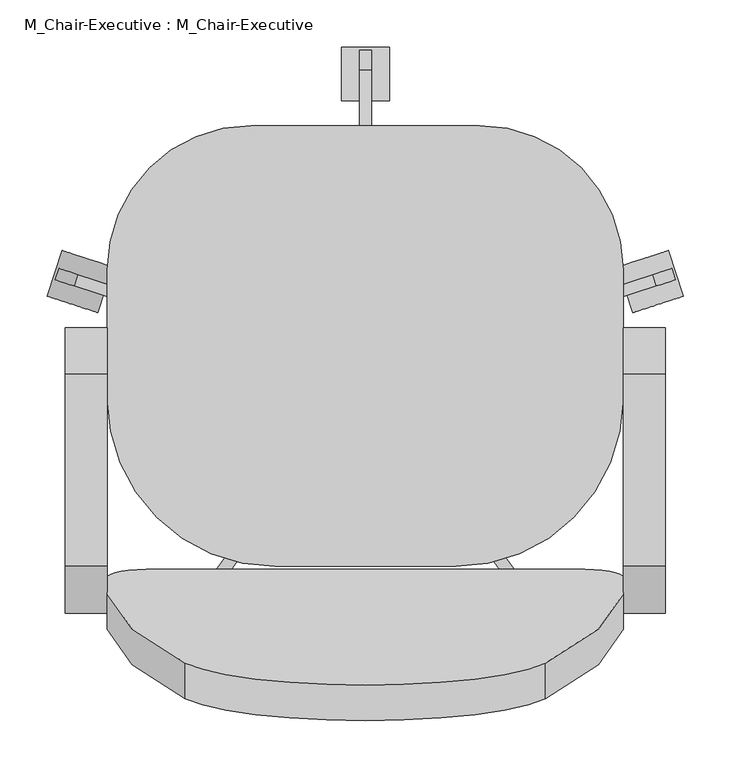
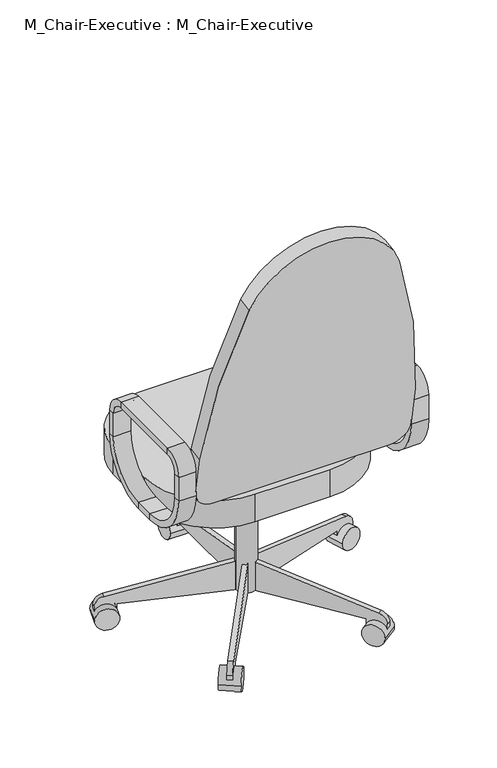
"""IFC4 building model written with IfcOpenShell, lengths in millimetres: furniture geometry, M_Chair-Executive : M_Chair-Executive."""

import ifcopenshell
import ifcopenshell.guid

model = None  # the IFC model being written
_history = None  # IfcOwnerHistory: only IFC2X3 demands one
_inside = {}  # id of a spatial element -> (the spatial element, [elements in it])
_under = {}  # id of a project, library or spatial element -> (it, [spatial elements below it])
_declared = {}  # id of a project -> (the project, [libraries it declares])
_typed = {}  # id of a type object -> (the type object, [elements of that type])
_made_of = {}  # id of a material, layer set ... -> (it, [elements and type objects made of it])


def new_model(schema):
    """Start an empty IFC model of exactly this schema.

    Asked for "IFC4X3", IfcOpenShell would pick the latest addendum, in which some entities
    have other attributes; the version numbers below select the first issue.
    IFC2X3 requires an IfcOwnerHistory on every rooted entity: one is made here for all.
    """
    global model, _history
    if schema == "IFC4X3":
        model = ifcopenshell.file(schema_version=(4, 3, 0, 0))
    else:
        model = ifcopenshell.file(schema=schema)
    _inside.clear()
    _under.clear()
    _declared.clear()
    _typed.clear()
    _made_of.clear()
    _history = None
    if model.schema == "IFC2X3":
        org = make("IfcOrganization", Name="unknown")
        user = make(
            "IfcPersonAndOrganization",
            ThePerson=make("IfcPerson", FamilyName="unknown"),
            TheOrganization=org,
        )
        app = make(
            "IfcApplication",
            ApplicationDeveloper=org,
            Version="unknown",
            ApplicationFullName="unknown",
            ApplicationIdentifier="unknown",
        )
        _history = make(
            "IfcOwnerHistory",
            OwningUser=user,
            OwningApplication=app,
            ChangeAction="ADDED",
            CreationDate=0,
        )
    return model


def make(cls, **values):
    """One entity of the class cls with the attributes given. An attribute that is None is left unset."""
    return model.create_entity(
        cls, **{name: value for name, value in values.items() if value is not None}
    )


def rooted(cls, **values):
    """An entity with a GlobalId (a new one), such as an element, a storey or a relation."""
    return make(cls, GlobalId=ifcopenshell.guid.new(), OwnerHistory=_history, **values)


def si_unit(unit_type, name, prefix=None):
    """IfcSIUnit, for example si_unit("LENGTHUNIT", "METRE", prefix="MILLI")."""
    return make("IfcSIUnit", UnitType=unit_type, Prefix=prefix, Name=name)


def assignment(units):
    """IfcUnitAssignment: the units of a project."""
    return None if units is None else make("IfcUnitAssignment", Units=units)


def point(xyz):
    """IfcCartesianPoint."""
    return None if xyz is None else make("IfcCartesianPoint", Coordinates=xyz)


def direction(xyz):
    """IfcDirection."""
    return None if xyz is None else make("IfcDirection", DirectionRatios=xyz)


def frame(location, z_axis=None, x_axis=None):
    """IfcAxis2Placement3D, a coordinate frame: its origin and axes. An axis left out is left unset."""
    return make(
        "IfcAxis2Placement3D",
        Location=point(location),
        Axis=direction(z_axis),
        RefDirection=direction(x_axis),
    )


def frame_2d(location, x_axis=None):
    """IfcAxis2Placement2D, a coordinate frame in the plane: its origin and x axis."""
    return make(
        "IfcAxis2Placement2D", Location=point(location), RefDirection=direction(x_axis)
    )


def origin():
    """The frame at (0, 0, 0) with its axes left unset."""
    return frame((0.0, 0.0, 0.0))


def place(relative_to, where):
    """IfcLocalPlacement: puts the frame where relative to a parent placement (None: the world)."""
    return make(
        "IfcLocalPlacement", PlacementRelTo=relative_to, RelativePlacement=where
    )


def context(
    kind, dimensions, precision=None, world=None, true_north=None, identifier=None
):
    """IfcGeometricRepresentationContext, for example the 3D "Model" context."""
    return make(
        "IfcGeometricRepresentationContext",
        ContextIdentifier=identifier,
        ContextType=kind,
        CoordinateSpaceDimension=dimensions,
        Precision=precision,
        WorldCoordinateSystem=world,
        TrueNorth=true_north,
    )


def project(units=None, contexts=None):
    """IfcProject with its units and contexts."""
    return rooted(
        "IfcProject",
        Name="project",
        RepresentationContexts=contexts,
        UnitsInContext=assignment(units),
    )


def spatial(cls, under=None, at=None, **own):
    """A site, building, storey or space (cls), placed at a placement, below another one or the project."""
    s = rooted(cls, ObjectPlacement=at, **own)
    if under is not None:
        _under.setdefault(under.id(), (under, []))[1].append(s)
    return s


def polyline(points):
    """IfcPolyline through the points."""
    return make("IfcPolyline", Points=[point(p) for p in points])


def circle_curve(where, radius):
    """IfcCircle in the frame where."""
    return make("IfcCircle", Position=where, Radius=radius)


def trimmed(basis, trim1, trim2, sense, master):
    """IfcTrimmedCurve: the piece of a basis curve between two trims."""
    return make(
        "IfcTrimmedCurve",
        BasisCurve=basis,
        Trim1=trim1,
        Trim2=trim2,
        SenseAgreement=sense,
        MasterRepresentation=master,
    )


def segment(curve, same_sense, transition):
    """IfcCompositeCurveSegment."""
    return make(
        "IfcCompositeCurveSegment",
        Transition=transition,
        SameSense=same_sense,
        ParentCurve=curve,
    )


def composite_curve(segments, self_intersect=None):
    """IfcCompositeCurve: segments joined end to end."""
    return make("IfcCompositeCurve", Segments=segments, SelfIntersect=self_intersect)


def outline(outer, holes=None, kind="AREA"):
    """IfcArbitraryClosedProfileDef: a profile drawn as a closed curve; with holes, ...WithVoids."""
    if holes is None:
        return make("IfcArbitraryClosedProfileDef", ProfileType=kind, OuterCurve=outer)
    return make(
        "IfcArbitraryProfileDefWithVoids",
        ProfileType=kind,
        OuterCurve=outer,
        InnerCurves=holes,
    )


def extrude(swept, where, along, depth):
    """IfcExtrudedAreaSolid: the profile swept, set in the frame where, extruded along a direction by depth."""
    return make(
        "IfcExtrudedAreaSolid",
        SweptArea=swept,
        Position=where,
        ExtrudedDirection=direction(along),
        Depth=depth,
    )


def shape(context_of_items, identifier, shape_type, items):
    """IfcShapeRepresentation: the items that make up one representation, for example the "Body"."""
    return make(
        "IfcShapeRepresentation",
        ContextOfItems=context_of_items,
        RepresentationIdentifier=identifier,
        RepresentationType=shape_type,
        Items=items,
    )


def source(mapping_origin, context_of_items, identifier, shape_type, items):
    """IfcRepresentationMap: a shape defined once, which mapped items show again and again."""
    return make(
        "IfcRepresentationMap",
        MappingOrigin=mapping_origin,
        MappedRepresentation=shape(context_of_items, identifier, shape_type, items),
    )


def transform(
    local_origin,
    x_axis=None,
    y_axis=None,
    z_axis=None,
    scale=None,
    scale2=None,
    scale3=None,
    uniform=True,
):
    """IfcCartesianTransformationOperator3D, or its non-uniform kind. x_axis, y_axis, z_axis: its Axis1, 2, 3."""
    if uniform:
        return make(
            "IfcCartesianTransformationOperator3D",
            Axis1=direction(x_axis),
            Axis2=direction(y_axis),
            LocalOrigin=point(local_origin),
            Scale=scale,
            Axis3=direction(z_axis),
        )
    return make(
        "IfcCartesianTransformationOperator3DnonUniform",
        Axis1=direction(x_axis),
        Axis2=direction(y_axis),
        LocalOrigin=point(local_origin),
        Scale=scale,
        Axis3=direction(z_axis),
        Scale2=scale2,
        Scale3=scale3,
    )


def mapped(mapping_source, mapping_target):
    """IfcMappedItem: shows the shape of a source again, moved by a transform."""
    return make(
        "IfcMappedItem", MappingSource=mapping_source, MappingTarget=mapping_target
    )


def made_of(thing, what):
    """Note that an element or type object is made of a material, layer set ...; save() writes the relation."""
    if what is not None:
        _made_of.setdefault(what.id(), (what, []))[1].append(thing)
    return thing


def element(
    cls,
    number,
    at=None,
    inside=None,
    cuts=None,
    type_object=None,
    material=None,
    context=None,
    identifier="Body",
    shape_type=None,
    held_by="IfcProductDefinitionShape",
    body=None,
    shapes=None,
    **own,
):
    """One element of the class cls, such as IfcWall. Its Tag is "e" and its number.

    at: its placement. inside: the storey or other place that contains it. cuts: it is an
    opening in that element (IfcRelVoidsElement). A single representation is given by context,
    identifier, shape_type and body (its items); several are given by shapes. held_by: the class
    of the entity that holds the representations. save() writes the other relations.
    """
    e = rooted(cls, Tag="e%d" % number, ObjectPlacement=at, **own)
    if body is not None:
        shapes = [shape(context, identifier, shape_type, body)]
    if shapes is not None:
        e.Representation = make(held_by, Representations=shapes)
    if inside is not None:
        _inside.setdefault(inside.id(), (inside, []))[1].append(e)
    if cuts is not None:
        rooted(
            "IfcRelVoidsElement", RelatingBuildingElement=cuts, RelatedOpeningElement=e
        )
    if type_object is not None:
        _typed.setdefault(type_object.id(), (type_object, []))[1].append(e)
    return made_of(e, material)


def aggregate(whole, parts):
    """IfcRelAggregates: a whole, such as a stair, and the parts it consists of."""
    return rooted("IfcRelAggregates", RelatingObject=whole, RelatedObjects=parts)


def save(model, path):
    """Write the relations noted so far, then the file.

    IfcRelAggregates (storeys below a building ...), IfcRelContainedInSpatialStructure (elements
    in a storey), IfcRelDefinesByType, IfcRelAssociatesMaterial and IfcRelDeclares: one each for
    every whole, place, type object, material and project.
    """
    for whole, parts in _under.values():
        aggregate(whole, parts)
    for where, things in _inside.values():
        rooted(
            "IfcRelContainedInSpatialStructure",
            RelatedElements=things,
            RelatingStructure=where,
        )
    for kind, things in _typed.values():
        rooted("IfcRelDefinesByType", RelatedObjects=things, RelatingType=kind)
    for what, things in _made_of.values():
        rooted("IfcRelAssociatesMaterial", RelatedObjects=things, RelatingMaterial=what)
    for by, libraries in _declared.values():
        rooted("IfcRelDeclares", RelatingContext=by, RelatedDefinitions=libraries)
    model.write(path)


def plane_surface(at):
    """IfcPlane: the flat surface through the origin of the frame at, square to its z axis."""
    return make("IfcPlane", Position=at)


def cylinder_surface(at, radius):
    """IfcCylindricalSurface: all points at the distance radius from the z axis of the frame at."""
    return make("IfcCylindricalSurface", Position=at, Radius=radius)


def revolved_surface(curve, axis_point, axis_direction):
    """IfcSurfaceOfRevolution: the curve turned about the line through axis_point along axis_direction."""
    return make(
        "IfcSurfaceOfRevolution",
        SweptCurve=make("IfcArbitraryOpenProfileDef", ProfileType="CURVE", Curve=curve),
        AxisPosition=make("IfcAxis1Placement", Location=point(axis_point), Axis=direction(axis_direction)),
    )


def advanced_brep(points, edges, surfaces, faces):
    """IfcAdvancedBrep: a solid bounded by faces that lie on surfaces and meet in shared edges.

    An edge is (start, end): straight between two places in points (the first is 0);
    or (start, end, curve); or (start, end, curve, False) where it runs against its curve.
    A face is (place in surfaces, loops), or (place, loops, False) where it looks against
    its surface's normal. A loop lists edges by number (the first is 1), with a minus sign
    where the edge is run from its end to its start. The first loop is the outer one.
    """
    corners = [point(p) for p in points]
    vertices = [make("IfcVertexPoint", VertexGeometry=c) for c in corners]
    made = []
    for start, end, *more in edges:
        made.append(
            make(
                "IfcEdgeCurve",
                EdgeStart=vertices[start],
                EdgeEnd=vertices[end],
                EdgeGeometry=more[0] if more else make("IfcPolyline", Points=[corners[start], corners[end]]),
                SameSense=more[1] if len(more) > 1 else True,
            )
        )
    hull = []
    for where, loops, *sense in faces:
        bounds = []
        for j, loop in enumerate(loops):
            ring = [make("IfcOrientedEdge", EdgeElement=made[abs(k) - 1], Orientation=k > 0) for k in loop]
            bounds.append(
                make(
                    "IfcFaceOuterBound" if j == 0 else "IfcFaceBound",
                    Bound=make("IfcEdgeLoop", EdgeList=ring),
                    Orientation=True,
                )
            )
        hull.append(make("IfcAdvancedFace", Bounds=bounds, FaceSurface=surfaces[where], SameSense=sense[0] if sense else True))
    return make("IfcAdvancedBrep", Outer=make("IfcClosedShell", CfsFaces=hull))


def m_chair_executive_m_chair_executive_8d69e98c(model_context):
    return source(origin(), model_context, "Body", "SolidModel", [
        advanced_brep(
        [(-176.5091803, -217.7873012, 546.1), (-176.5091803, -108.0540984, 436.3667972), (-176.5091803, -108.0540984, 420.4917972), (-176.5091803, -233.6623012, 546.1), (-132.0591803, -217.7873012, 546.1), (-132.0591803, -108.0540984, 436.3667972), (-132.0591803, -233.6623012, 546.1), (-132.0591803, -108.0540984, 420.4917972), (-176.5091803, -233.6623012, 609.6), (-176.5091803, -217.7873012, 609.6), (-132.0591803, -217.7873012, 609.6), (-132.0591803, -233.6623012, 609.6), (-176.5091803, -184.2540984, 643.1332028), (-176.5091803, -184.2540984, 659.0082028), (-132.0591803, -184.2540984, 643.1332028), (-132.0591803, -184.2540984, 659.0082028), (-176.5091803, 18.9459016, 659.0082028), (-176.5091803, 18.9459016, 643.1332028), (-132.0591803, 18.9459016, 643.1332028), (-132.0591803, 18.9459016, 659.0082028), (-176.5091803, 52.4791044, 609.6), (-176.5091803, 68.3541044, 609.6), (-132.0591803, 52.4791044, 609.6), (-132.0591803, 68.3541044, 609.6), (-176.5091803, 68.3541044, 546.1), (-176.5091803, 52.4791044, 546.1), (-132.0591803, 52.4791044, 546.1), (-132.0591803, 68.3541044, 546.1), (-176.5091803, -57.2540984, 436.3667972), (-176.5091803, -57.2540984, 420.4917972), (-132.0591803, -57.2540984, 436.3667972), (-132.0591803, -57.2540984, 420.4917972)],
        [
            (0, 1, circle_curve(frame((-176.5091803, -108.0540984, 546.1), z_axis=(1.0, 0.0, 0.0), x_axis=(0.0, 0.0, -1.0)), 109.7332028)),
            (1, 2),
            (2, 3, circle_curve(frame((-176.5091803, -108.0540984, 546.1), z_axis=(-1.0, 0.0, 0.0), x_axis=(0.0, 0.0, -1.0)), 125.6082028)),
            (3, 0),
            (4, 5, circle_curve(frame((-132.0591803, -108.0540984, 546.1), z_axis=(1.0, 0.0, 0.0), x_axis=(0.0, 0.0, -1.0)), 109.7332028)),
            (5, 1),
            (0, 4),
            (6, 7, circle_curve(frame((-132.0591803, -108.0540984, 546.1), z_axis=(1.0, 0.0, 0.0), x_axis=(0.0, 0.0, -1.0)), 125.6082028)),
            (7, 5),
            (4, 6),
            (2, 7),
            (6, 3),
            (3, 8),
            (8, 9),
            (9, 0),
            (9, 10),
            (10, 4),
            (10, 11),
            (11, 6),
            (11, 8),
            (12, 9, circle_curve(frame((-176.5091803, -184.2540984, 609.6), z_axis=(1.0, 0.0, 0.0), x_axis=(0.0, -1.0, 0.0)), 33.5332028)),
            (8, 13, circle_curve(frame((-176.5091803, -184.2540984, 609.6), z_axis=(-1.0, 0.0, 0.0), x_axis=(0.0, -1.0, 0.0)), 49.4082028)),
            (13, 12),
            (14, 10, circle_curve(frame((-132.0591803, -184.2540984, 609.6), z_axis=(1.0, 0.0, 0.0), x_axis=(0.0, -1.0, 0.0)), 33.5332028)),
            (12, 14),
            (15, 11, circle_curve(frame((-132.0591803, -184.2540984, 609.6), z_axis=(1.0, 0.0, 0.0), x_axis=(0.0, -1.0, 0.0)), 49.4082028)),
            (14, 15),
            (15, 13),
            (13, 16),
            (16, 17),
            (17, 12),
            (17, 18),
            (18, 14),
            (18, 19),
            (19, 15),
            (19, 16),
            (20, 17, circle_curve(frame((-176.5091803, 18.9459016, 609.6), z_axis=(1.0, 0.0, 0.0), x_axis=(0.0, 0.0, 1.0)), 33.5332028)),
            (16, 21, circle_curve(frame((-176.5091803, 18.9459016, 609.6), z_axis=(-1.0, 0.0, 0.0), x_axis=(0.0, 0.0, 1.0)), 49.4082028)),
            (21, 20),
            (22, 18, circle_curve(frame((-132.0591803, 18.9459016, 609.6), z_axis=(1.0, 0.0, 0.0), x_axis=(0.0, 0.0, 1.0)), 33.5332028)),
            (20, 22),
            (23, 19, circle_curve(frame((-132.0591803, 18.9459016, 609.6), z_axis=(1.0, 0.0, 0.0), x_axis=(0.0, 0.0, 1.0)), 49.4082028)),
            (22, 23),
            (23, 21),
            (21, 24),
            (24, 25),
            (25, 20),
            (25, 26),
            (26, 22),
            (26, 27),
            (27, 23),
            (27, 24),
            (28, 25, circle_curve(frame((-176.5091803, -57.2540984, 546.1), z_axis=(1.0, 0.0, 0.0), x_axis=(0.0, 1.0, 0.0)), 109.7332028)),
            (24, 29, circle_curve(frame((-176.5091803, -57.2540984, 546.1), z_axis=(-1.0, 0.0, 0.0), x_axis=(0.0, 1.0, 0.0)), 125.6082028)),
            (29, 28),
            (30, 26, circle_curve(frame((-132.0591803, -57.2540984, 546.1), z_axis=(1.0, 0.0, 0.0), x_axis=(0.0, 1.0, 0.0)), 109.7332028)),
            (28, 30),
            (31, 27, circle_curve(frame((-132.0591803, -57.2540984, 546.1), z_axis=(1.0, 0.0, 0.0), x_axis=(0.0, 1.0, 0.0)), 125.6082028)),
            (30, 31),
            (31, 29),
            (29, 2),
            (1, 28),
            (5, 30),
            (7, 31),
        ],
        [
            plane_surface(frame((-176.5091803, -108.0540984, 546.1), z_axis=(-1.0, 0.0, 0.0), x_axis=(0.0, 0.0, -1.0))),
            revolved_surface(polyline([(-176.5091803, -108.0540984, 436.3667972), (-132.0591803, -108.0540984, 436.3667972)]), (-132.0591803, -108.0540984, 546.1), (-1.0, 0.0, 0.0)),
            plane_surface(frame((-132.0591803, -108.0540984, 546.1), z_axis=(1.0, 0.0, 0.0), x_axis=(0.0, 0.0, -1.0))),
            cylinder_surface(frame((-132.0591803, -108.0540984, 546.1), z_axis=(-1.0, 0.0, 0.0), x_axis=(0.0, 0.0, -1.0)), 125.6082028),
            plane_surface(frame((-176.5091803, -233.6623012, 546.1), z_axis=(-1.0, 0.0, 0.0), x_axis=(0.0, 0.0, 1.0))),
            plane_surface(frame((-176.5091803, -217.7873012, 546.1), z_axis=(0.0, 1.0, 0.0), x_axis=(0.0, 0.0, 1.0))),
            plane_surface(frame((-132.0591803, -217.7873012, 546.1), z_axis=(1.0, 0.0, 0.0), x_axis=(0.0, 0.0, 1.0))),
            plane_surface(frame((-132.0591803, -233.6623012, 546.1), z_axis=(0.0, -1.0, 0.0), x_axis=(0.0, 0.0, 1.0))),
            plane_surface(frame((-176.5091803, -184.2540984, 609.6), z_axis=(-1.0, 0.0, 0.0), x_axis=(0.0, -1.0, 0.0))),
            revolved_surface(polyline([(-176.5091803, -217.7873012, 609.6), (-132.0591803, -217.7873012, 609.6)]), (-132.0591803, -184.2540984, 609.6), (-1.0, 0.0, 0.0)),
            plane_surface(frame((-132.0591803, -184.2540984, 609.6), z_axis=(1.0, 0.0, 0.0), x_axis=(0.0, -1.0, 0.0))),
            cylinder_surface(frame((-132.0591803, -184.2540984, 609.6), z_axis=(-1.0, 0.0, 0.0), x_axis=(0.0, -1.0, 0.0)), 49.4082028),
            plane_surface(frame((-176.5091803, -184.2540984, 659.0082028), z_axis=(-1.0, 0.0, 0.0), x_axis=(0.0, 1.0, 0.0))),
            plane_surface(frame((-176.5091803, -184.2540984, 643.1332028), z_axis=(0.0, 0.0, -1.0), x_axis=(0.0, 1.0, 0.0))),
            plane_surface(frame((-132.0591803, -184.2540984, 643.1332028), z_axis=(1.0, 0.0, 0.0), x_axis=(0.0, 1.0, 0.0))),
            plane_surface(frame((-132.0591803, -184.2540984, 659.0082028), z_axis=(0.0, 0.0, 1.0), x_axis=(0.0, 1.0, 0.0))),
            plane_surface(frame((-176.5091803, 18.9459016, 609.6), z_axis=(-1.0, 0.0, 0.0), x_axis=(0.0, 0.0, 1.0))),
            revolved_surface(polyline([(-176.5091803, 18.9459016, 643.1332028), (-132.0591803, 18.9459016, 643.1332028)]), (-132.0591803, 18.9459016, 609.6), (-1.0, 0.0, 0.0)),
            plane_surface(frame((-132.0591803, 18.9459016, 609.6), z_axis=(1.0, 0.0, 0.0), x_axis=(0.0, 0.0, 1.0))),
            cylinder_surface(frame((-132.0591803, 18.9459016, 609.6), z_axis=(-1.0, 0.0, 0.0), x_axis=(0.0, 0.0, 1.0)), 49.4082028),
            plane_surface(frame((-176.5091803, 68.3541044, 609.6), z_axis=(-1.0, 0.0, 0.0), x_axis=(0.0, 0.0, -1.0))),
            plane_surface(frame((-176.5091803, 52.4791044, 609.6), z_axis=(0.0, -1.0, 0.0), x_axis=(0.0, 0.0, -1.0))),
            plane_surface(frame((-132.0591803, 52.4791044, 609.6), z_axis=(1.0, 0.0, 0.0), x_axis=(0.0, 0.0, -1.0))),
            plane_surface(frame((-132.0591803, 68.3541044, 609.6), z_axis=(0.0, 1.0, 0.0), x_axis=(0.0, 0.0, -1.0))),
            plane_surface(frame((-176.5091803, -57.2540984, 546.1), z_axis=(-1.0, 0.0, 0.0), x_axis=(0.0, 1.0, 0.0))),
            revolved_surface(polyline([(-176.5091803, 52.479104400000004, 546.1), (-132.0591803, 52.479104400000004, 546.1)]), (-132.0591803, -57.2540984, 546.1), (-1.0, 0.0, 0.0)),
            plane_surface(frame((-132.0591803, -57.2540984, 546.1), z_axis=(1.0, 0.0, 0.0), x_axis=(0.0, 1.0, 0.0))),
            cylinder_surface(frame((-132.0591803, -57.2540984, 546.1), z_axis=(-1.0, 0.0, 0.0), x_axis=(0.0, 1.0, 0.0)), 125.6082028),
            plane_surface(frame((-176.5091803, -57.2540984, 420.4917972), z_axis=(-1.0, 0.0, 0.0), x_axis=(0.0, -1.0, 0.0))),
            plane_surface(frame((-176.5091803, -57.2540984, 436.3667972), z_axis=(0.0, 0.0, 1.0), x_axis=(0.0, -1.0, 0.0))),
            plane_surface(frame((-132.0591803, -57.2540984, 436.3667972), z_axis=(1.0, 0.0, 0.0), x_axis=(0.0, -1.0, 0.0))),
            plane_surface(frame((-132.0591803, -57.2540984, 420.4917972), z_axis=(0.0, 0.0, -1.0), x_axis=(0.0, -1.0, 0.0))),
        ],
        [
            (0, [[1, 2, 3, 4]]),
            (1, [[5, 6, -1, 7]]),
            (2, [[8, 9, -5, 10]]),
            (3, [[-3, 11, -8, 12]]),
            (4, [[-4, 13, 14, 15]]),
            (5, [[-7, -15, 16, 17]]),
            (6, [[-10, -17, 18, 19]]),
            (7, [[-12, -19, 20, -13]]),
            (8, [[21, -14, 22, 23]]),
            (9, [[24, -16, -21, 25]]),
            (10, [[26, -18, -24, 27]]),
            (11, [[-22, -20, -26, 28]]),
            (12, [[-23, 29, 30, 31]]),
            (13, [[-25, -31, 32, 33]]),
            (14, [[-27, -33, 34, 35]]),
            (15, [[-28, -35, 36, -29]]),
            (16, [[37, -30, 38, 39]]),
            (17, [[40, -32, -37, 41]]),
            (18, [[42, -34, -40, 43]]),
            (19, [[-38, -36, -42, 44]]),
            (20, [[-39, 45, 46, 47]]),
            (21, [[-41, -47, 48, 49]]),
            (22, [[-43, -49, 50, 51]]),
            (23, [[-44, -51, 52, -45]]),
            (24, [[53, -46, 54, 55]]),
            (25, [[56, -48, -53, 57]]),
            (26, [[58, -50, -56, 59]]),
            (27, [[-54, -52, -58, 60]]),
            (28, [[-55, 61, -2, 62]]),
            (29, [[-57, -62, -6, 63]]),
            (30, [[-59, -63, -9, 64]]),
            (31, [[-60, -64, -11, -61]]),
        ],
    ),
        advanced_brep(
        [(414.0408197, -233.6623012, 546.1), (414.0408197, -108.0540984, 420.4917972), (458.4908197, -108.0540984, 420.4917972), (458.4908197, -233.6623012, 546.1), (414.0408197, -217.7873012, 546.1), (414.0408197, -108.0540984, 436.3667972), (458.4908197, -217.7873012, 546.1), (458.4908197, -108.0540984, 436.3667972), (458.4908197, -233.6623012, 609.6), (414.0408197, -233.6623012, 609.6), (414.0408197, -217.7873012, 609.6), (458.4908197, -217.7873012, 609.6), (414.0408197, -184.2540984, 659.0082028), (458.4908197, -184.2540984, 659.0082028), (414.0408197, -184.2540984, 643.1332028), (458.4908197, -184.2540984, 643.1332028), (458.4908197, 18.9459016, 659.0082028), (414.0408197, 18.9459016, 659.0082028), (414.0408197, 18.9459016, 643.1332028), (458.4908197, 18.9459016, 643.1332028), (414.0408197, 68.3541044, 609.6), (458.4908197, 68.3541044, 609.6), (414.0408197, 52.4791044, 609.6), (458.4908197, 52.4791044, 609.6), (458.4908197, 68.3541044, 546.1), (414.0408197, 68.3541044, 546.1), (414.0408197, 52.4791044, 546.1), (458.4908197, 52.4791044, 546.1), (414.0408197, -57.2540984, 420.4917972), (458.4908197, -57.2540984, 420.4917972), (414.0408197, -57.2540984, 436.3667972), (458.4908197, -57.2540984, 436.3667972)],
        [
            (0, 1, circle_curve(frame((414.0408197, -108.0540984, 546.1), z_axis=(1.0, 0.0, 0.0), x_axis=(0.0, 0.0, -1.0)), 125.6082028)),
            (1, 2),
            (2, 3, circle_curve(frame((458.4908197, -108.0540984, 546.1), z_axis=(-1.0, 0.0, 0.0), x_axis=(0.0, 0.0, -1.0)), 125.6082028)),
            (3, 0),
            (4, 5, circle_curve(frame((414.0408197, -108.0540984, 546.1), z_axis=(1.0, 0.0, 0.0), x_axis=(0.0, 0.0, -1.0)), 109.7332028)),
            (5, 1),
            (0, 4),
            (6, 7, circle_curve(frame((458.4908197, -108.0540984, 546.1), z_axis=(1.0, 0.0, 0.0), x_axis=(0.0, 0.0, -1.0)), 109.7332028)),
            (7, 5),
            (4, 6),
            (2, 7),
            (6, 3),
            (3, 8),
            (8, 9),
            (9, 0),
            (9, 10),
            (10, 4),
            (10, 11),
            (11, 6),
            (11, 8),
            (12, 9, circle_curve(frame((414.0408197, -184.2540984, 609.6), z_axis=(1.0, 0.0, 0.0), x_axis=(0.0, -1.0, 0.0)), 49.4082028)),
            (8, 13, circle_curve(frame((458.4908197, -184.2540984, 609.6), z_axis=(-1.0, 0.0, 0.0), x_axis=(0.0, -1.0, 0.0)), 49.4082028)),
            (13, 12),
            (14, 10, circle_curve(frame((414.0408197, -184.2540984, 609.6), z_axis=(1.0, 0.0, 0.0), x_axis=(0.0, -1.0, 0.0)), 33.5332028)),
            (12, 14),
            (15, 11, circle_curve(frame((458.4908197, -184.2540984, 609.6), z_axis=(1.0, 0.0, 0.0), x_axis=(0.0, -1.0, 0.0)), 33.5332028)),
            (14, 15),
            (15, 13),
            (13, 16),
            (16, 17),
            (17, 12),
            (17, 18),
            (18, 14),
            (18, 19),
            (19, 15),
            (19, 16),
            (20, 17, circle_curve(frame((414.0408197, 18.9459016, 609.6), z_axis=(1.0, 0.0, 0.0), x_axis=(0.0, 0.0, 1.0)), 49.4082028)),
            (16, 21, circle_curve(frame((458.4908197, 18.9459016, 609.6), z_axis=(-1.0, 0.0, 0.0), x_axis=(0.0, 0.0, 1.0)), 49.4082028)),
            (21, 20),
            (22, 18, circle_curve(frame((414.0408197, 18.9459016, 609.6), z_axis=(1.0, 0.0, 0.0), x_axis=(0.0, 0.0, 1.0)), 33.5332028)),
            (20, 22),
            (23, 19, circle_curve(frame((458.4908197, 18.9459016, 609.6), z_axis=(1.0, 0.0, 0.0), x_axis=(0.0, 0.0, 1.0)), 33.5332028)),
            (22, 23),
            (23, 21),
            (21, 24),
            (24, 25),
            (25, 20),
            (25, 26),
            (26, 22),
            (26, 27),
            (27, 23),
            (27, 24),
            (28, 25, circle_curve(frame((414.0408197, -57.2540984, 546.1), z_axis=(1.0, 0.0, 0.0), x_axis=(0.0, 1.0, 0.0)), 125.6082028)),
            (24, 29, circle_curve(frame((458.4908197, -57.2540984, 546.1), z_axis=(-1.0, 0.0, 0.0), x_axis=(0.0, 1.0, 0.0)), 125.6082028)),
            (29, 28),
            (30, 26, circle_curve(frame((414.0408197, -57.2540984, 546.1), z_axis=(1.0, 0.0, 0.0), x_axis=(0.0, 1.0, 0.0)), 109.7332028)),
            (28, 30),
            (31, 27, circle_curve(frame((458.4908197, -57.2540984, 546.1), z_axis=(1.0, 0.0, 0.0), x_axis=(0.0, 1.0, 0.0)), 109.7332028)),
            (30, 31),
            (31, 29),
            (29, 2),
            (1, 28),
            (5, 30),
            (7, 31),
        ],
        [
            cylinder_surface(frame((414.0408197, -108.0540984, 546.1), z_axis=(-1.0, 0.0, 0.0), x_axis=(0.0, 0.0, -1.0)), 125.6082028),
            plane_surface(frame((414.0408197, -108.0540984, 546.1), z_axis=(-1.0, 0.0, 0.0), x_axis=(0.0, 0.0, -1.0))),
            revolved_surface(polyline([(414.0408197, -108.0540984, 436.3667972), (458.4908197, -108.0540984, 436.3667972)]), (414.0408197, -108.0540984, 546.1), (-1.0, 0.0, 0.0)),
            plane_surface(frame((458.4908197, -108.0540984, 546.1), z_axis=(1.0, 0.0, 0.0), x_axis=(0.0, 0.0, -1.0))),
            plane_surface(frame((458.4908197, -233.6623012, 546.1), z_axis=(0.0, -1.0, 0.0), x_axis=(0.0, 0.0, 1.0))),
            plane_surface(frame((414.0408197, -233.6623012, 546.1), z_axis=(-1.0, 0.0, 0.0), x_axis=(0.0, 0.0, 1.0))),
            plane_surface(frame((414.0408197, -217.7873012, 546.1), z_axis=(0.0, 1.0, 0.0), x_axis=(0.0, 0.0, 1.0))),
            plane_surface(frame((458.4908197, -217.7873012, 546.1), z_axis=(1.0, 0.0, 0.0), x_axis=(0.0, 0.0, 1.0))),
            cylinder_surface(frame((414.0408197, -184.2540984, 609.6), z_axis=(-1.0, 0.0, 0.0), x_axis=(0.0, -1.0, 0.0)), 49.4082028),
            plane_surface(frame((414.0408197, -184.2540984, 609.6), z_axis=(-1.0, 0.0, 0.0), x_axis=(0.0, -1.0, 0.0))),
            revolved_surface(polyline([(414.0408197, -217.7873012, 609.6), (458.4908197, -217.7873012, 609.6)]), (414.0408197, -184.2540984, 609.6), (-1.0, 0.0, 0.0)),
            plane_surface(frame((458.4908197, -184.2540984, 609.6), z_axis=(1.0, 0.0, 0.0), x_axis=(0.0, -1.0, 0.0))),
            plane_surface(frame((458.4908197, -184.2540984, 659.0082028), z_axis=(0.0, 0.0, 1.0), x_axis=(0.0, 1.0, 0.0))),
            plane_surface(frame((414.0408197, -184.2540984, 659.0082028), z_axis=(-1.0, 0.0, 0.0), x_axis=(0.0, 1.0, 0.0))),
            plane_surface(frame((414.0408197, -184.2540984, 643.1332028), z_axis=(0.0, 0.0, -1.0), x_axis=(0.0, 1.0, 0.0))),
            plane_surface(frame((458.4908197, -184.2540984, 643.1332028), z_axis=(1.0, 0.0, 0.0), x_axis=(0.0, 1.0, 0.0))),
            cylinder_surface(frame((414.0408197, 18.9459016, 609.6), z_axis=(-1.0, 0.0, 0.0), x_axis=(0.0, 0.0, 1.0)), 49.4082028),
            plane_surface(frame((414.0408197, 18.9459016, 609.6), z_axis=(-1.0, 0.0, 0.0), x_axis=(0.0, 0.0, 1.0))),
            revolved_surface(polyline([(414.0408197, 18.9459016, 643.1332028), (458.4908197, 18.9459016, 643.1332028)]), (414.0408197, 18.9459016, 609.6), (-1.0, 0.0, 0.0)),
            plane_surface(frame((458.4908197, 18.9459016, 609.6), z_axis=(1.0, 0.0, 0.0), x_axis=(0.0, 0.0, 1.0))),
            plane_surface(frame((458.4908197, 68.3541044, 609.6), z_axis=(0.0, 1.0, 0.0), x_axis=(0.0, 0.0, -1.0))),
            plane_surface(frame((414.0408197, 68.3541044, 609.6), z_axis=(-1.0, 0.0, 0.0), x_axis=(0.0, 0.0, -1.0))),
            plane_surface(frame((414.0408197, 52.4791044, 609.6), z_axis=(0.0, -1.0, 0.0), x_axis=(0.0, 0.0, -1.0))),
            plane_surface(frame((458.4908197, 52.4791044, 609.6), z_axis=(1.0, 0.0, 0.0), x_axis=(0.0, 0.0, -1.0))),
            cylinder_surface(frame((414.0408197, -57.2540984, 546.1), z_axis=(-1.0, 0.0, 0.0), x_axis=(0.0, 1.0, 0.0)), 125.6082028),
            plane_surface(frame((414.0408197, -57.2540984, 546.1), z_axis=(-1.0, 0.0, 0.0), x_axis=(0.0, 1.0, 0.0))),
            revolved_surface(polyline([(414.0408197, 52.479104400000004, 546.1), (458.4908197, 52.479104400000004, 546.1)]), (414.0408197, -57.2540984, 546.1), (-1.0, 0.0, 0.0)),
            plane_surface(frame((458.4908197, -57.2540984, 546.1), z_axis=(1.0, 0.0, 0.0), x_axis=(0.0, 1.0, 0.0))),
            plane_surface(frame((458.4908197, -57.2540984, 420.4917972), z_axis=(0.0, 0.0, -1.0), x_axis=(0.0, -1.0, 0.0))),
            plane_surface(frame((414.0408197, -57.2540984, 420.4917972), z_axis=(-1.0, 0.0, 0.0), x_axis=(0.0, -1.0, 0.0))),
            plane_surface(frame((414.0408197, -57.2540984, 436.3667972), z_axis=(0.0, 0.0, 1.0), x_axis=(0.0, -1.0, 0.0))),
            plane_surface(frame((458.4908197, -57.2540984, 436.3667972), z_axis=(1.0, 0.0, 0.0), x_axis=(0.0, -1.0, 0.0))),
        ],
        [
            (0, [[1, 2, 3, 4]]),
            (1, [[5, 6, -1, 7]]),
            (2, [[8, 9, -5, 10]]),
            (3, [[-3, 11, -8, 12]]),
            (4, [[-4, 13, 14, 15]]),
            (5, [[-7, -15, 16, 17]]),
            (6, [[-10, -17, 18, 19]]),
            (7, [[-12, -19, 20, -13]]),
            (8, [[21, -14, 22, 23]]),
            (9, [[24, -16, -21, 25]]),
            (10, [[26, -18, -24, 27]]),
            (11, [[-22, -20, -26, 28]]),
            (12, [[-23, 29, 30, 31]]),
            (13, [[-25, -31, 32, 33]]),
            (14, [[-27, -33, 34, 35]]),
            (15, [[-28, -35, 36, -29]]),
            (16, [[37, -30, 38, 39]]),
            (17, [[40, -32, -37, 41]]),
            (18, [[42, -34, -40, 43]]),
            (19, [[-38, -36, -42, 44]]),
            (20, [[-39, 45, 46, 47]]),
            (21, [[-41, -47, 48, 49]]),
            (22, [[-43, -49, 50, 51]]),
            (23, [[-44, -51, 52, -45]]),
            (24, [[53, -46, 54, 55]]),
            (25, [[56, -48, -53, 57]]),
            (26, [[58, -50, -56, 59]]),
            (27, [[-54, -52, -58, 60]]),
            (28, [[-55, 61, -2, 62]]),
            (29, [[-57, -62, -6, 63]]),
            (30, [[-59, -63, -9, 64]]),
            (31, [[-60, -64, -11, -61]]),
        ],
    ),
        extrude(outline(composite_curve([segment(trimmed(circle_curve(frame_2d((0.0, -50.8)), 50.8), [point((0.0, 0.0))], [point((50.8, -50.8))], False, "CARTESIAN"), True, "CONTINUOUS"), segment(polyline([(50.8, -50.8), (50.8, -152.4)]), True, "CONTINUOUS"), segment(trimmed(circle_curve(frame_2d((-1471.2021854, -74.3913617)), 1524.0), [point((50.8, -152.4))], [point((-31.75, -574.9444618))], False, "CARTESIAN"), True, "CONTINUOUS"), segment(trimmed(circle_curve(frame_2d((-222.25, -504.2338544)), 203.2), [point((-31.75, -574.9444618))], [point((-412.75, -574.9444618))], False, "CARTESIAN"), True, "CONTINUOUS"), segment(trimmed(circle_curve(frame_2d((1026.7021854, -74.3913617)), 1524.0), [point((-412.75, -574.9444618))], [point((-495.3, -152.4))], False, "CARTESIAN"), True, "CONTINUOUS"), segment(polyline([(-495.3, -152.4), (-495.3, -50.8)]), True, "CONTINUOUS"), segment(trimmed(circle_curve(frame_2d((-444.5, -50.8)), 50.8), [point((-495.3, -50.8))], [point((-444.5, 0.0))], False, "CARTESIAN"), True, "CONTINUOUS"), segment(polyline([(-444.5, 0.0), (0.0, 0.0)]), True, "CONTINUOUS")], self_intersect=False)), frame((363.2408197, -224.5698964, 503.1641822), z_axis=(0.0, 0.9848077530122084, 0.17364817766692853), x_axis=(1.0, 0.0, 0.0)), (0.0, 0.0, 1.0), 38.1),
        extrude(outline(composite_curve([segment(trimmed(circle_curve(frame_2d((20.3408197, 129.4961016)), 152.4), [point((-132.0591803, 129.4961016))], [point((20.3408197, 281.8961016))], False, "CARTESIAN"), True, "CONTINUOUS"), segment(polyline([(20.3408197, 281.8961016), (261.6408197, 281.8961016)]), True, "CONTINUOUS"), segment(trimmed(circle_curve(frame_2d((261.6408197, 129.4961016)), 152.4), [point((261.6408197, 281.8961016))], [point((414.0408197, 129.4961016))], False, "CARTESIAN"), True, "CONTINUOUS"), segment(polyline([(414.0408197, 129.4961016), (414.0408197, -6.4540984)]), True, "CONTINUOUS"), segment(trimmed(circle_curve(frame_2d((236.2408197, -6.4540984)), 177.8), [point((414.0408197, -6.4540984))], [point((236.2408197, -184.2540984))], False, "CARTESIAN"), True, "CONTINUOUS"), segment(polyline([(236.2408197, -184.2540984), (45.7408197, -184.2540984)]), True, "CONTINUOUS"), segment(trimmed(circle_curve(frame_2d((45.7408197, -6.4540984)), 177.8), [point((45.7408197, -184.2540984))], [point((-132.0591803, -6.4540984))], False, "CARTESIAN"), True, "CONTINUOUS"), segment(polyline([(-132.0591803, -6.4540984), (-132.0591803, 129.4961016)]), True, "CONTINUOUS")], self_intersect=False)), frame((0.0, 0.0, 383.7835944), z_axis=(0.0, 0.0, 1.0), x_axis=(1.0, 0.0, 0.0)), (0.0, 0.0, 1.0), 73.4164056),
        extrude(outline(composite_curve([segment(trimmed(circle_curve(frame_2d((140.9908197, 18.9459016)), 25.4), [point((115.5908197, 18.9459016))], [point((166.3908197, 18.9459016))], False, "CARTESIAN"), True, "CONTINUOUS"), segment(trimmed(circle_curve(frame_2d((140.9908197, 18.9459016)), 25.4), [point((166.3908197, 18.9459016))], [point((115.5908197, 18.9459016))], False, "CARTESIAN"), True, "CONTINUOUS")], self_intersect=False)), frame((0.0, 0.0, 53.5835944), z_axis=(0.0, 0.0, 1.0), x_axis=(1.0, 0.0, 0.0)), (0.0, 0.0, 1.0), 330.5914056),
        extrude(outline(composite_curve([segment(trimmed(circle_curve(frame_2d((0.0, -28.2002727)), 28.2002727), [point((0.0, -56.4005455))], [point((0.0, 0.0))], False, "CARTESIAN"), True, "CONTINUOUS"), segment(trimmed(circle_curve(frame_2d((0.0, -28.2002727)), 28.2002727), [point((0.0, 0.0))], [point((0.0, -56.4005455))], False, "CARTESIAN"), True, "CONTINUOUS")], self_intersect=False)), frame((477.6203484, 101.6163254, 28.1835944), z_axis=(-0.3090169943749423, 0.9510565162951553, 0.0), x_axis=(0.0, 0.0, 1.0)), (0.0, 0.0, 1.0), 50.8),
        extrude(outline(composite_curve([segment(polyline([(-25.4, 0.0), (0.0, 0.0), (0.0, -50.8), (-24.303053, -50.8)]), True, "CONTINUOUS"), segment(trimmed(circle_curve(frame_2d((-24.303053, -25.4)), 25.4), [point((-24.303053, -50.8))], [point((-49.3171699, -29.8106637))], False, "CARTESIAN"), True, "CONTINUOUS"), segment(polyline([(-49.3171699, -29.8106637), (-101.6, 266.7), (-101.6, 292.1), (-25.4, 292.1), (-25.4, 0.0)]), True, "CONTINUOUS")], self_intersect=False)), frame((420.756686, 103.1705568, 28.1835944), z_axis=(-0.3090169943749423, 0.9510565162951553, 0.0), x_axis=(0.0, 0.0, -1.0)), (0.0, 0.0, 1.0), 12.7),
        extrude(outline(composite_curve([segment(trimmed(circle_curve(frame_2d((0.0, -28.2002727)), 28.2002727), [point((0.0, -56.4005455))], [point((0.0, 0.0))], False, "CARTESIAN"), True, "CONTINUOUS"), segment(trimmed(circle_curve(frame_2d((0.0, -28.2002727)), 28.2002727), [point((0.0, 0.0))], [point((0.0, -56.4005455))], False, "CARTESIAN"), True, "CONTINUOUS")], self_intersect=False)), frame((323.63931, -275.6612394, 28.1835944), z_axis=(0.8090169943749499, 0.5877852522924699, 0.0), x_axis=(0.0, 0.0, 1.0)), (0.0, 0.0, 1.0), 50.8),
        extrude(outline(composite_curve([segment(polyline([(-25.4, 0.0), (0.0, 0.0), (0.0, -50.8), (-24.303053, -50.8)]), True, "CONTINUOUS"), segment(trimmed(circle_curve(frame_2d((-24.303053, -25.3999999)), 25.4), [point((-24.303053, -50.8))], [point((-49.3171699, -29.8106636))], False, "CARTESIAN"), True, "CONTINUOUS"), segment(polyline([(-49.3171699, -29.8106636), (-101.6, 266.7), (-101.6, 292.1), (-25.4, 292.1), (-25.4, 0.0)]), True, "CONTINUOUS")], self_intersect=False)), frame((307.545634, -221.1003988, 28.1835944), z_axis=(0.8090169943749499, 0.5877852522924699, 0.0), x_axis=(0.0, 0.0, -1.0)), (0.0, 0.0, 1.0), 12.7),
        extrude(outline(composite_curve([segment(trimmed(circle_curve(frame_2d((0.0, -28.2002727)), 28.2002727), [point((0.0, -56.4005455))], [point((0.0, 0.0))], False, "CARTESIAN"), True, "CONTINUOUS"), segment(trimmed(circle_curve(frame_2d((0.0, -28.2002727)), 28.2002727), [point((0.0, 0.0))], [point((0.0, -56.4005455))], False, "CARTESIAN"), True, "CONTINUOUS")], self_intersect=False)), frame((-41.6576707, -275.6612394, 28.1835944), z_axis=(-0.8090169943749458, 0.5877852522924754, 0.0), x_axis=(0.0, 0.0, -1.0)), (0.0, 0.0, 1.0), 50.8),
        extrude(outline(composite_curve([segment(polyline([(25.4, 0.0), (25.4, 292.1), (101.6, 292.1), (101.6, 266.7), (49.3171699, -29.8106637)]), True, "CONTINUOUS"), segment(trimmed(circle_curve(frame_2d((24.303053, -25.3999999)), 25.4), [point((49.3171699, -29.8106637))], [point((24.303053, -50.8))], False, "CARTESIAN"), True, "CONTINUOUS"), segment(polyline([(24.303053, -50.8), (0.0, -50.8), (0.0, 0.0), (25.4, 0.0)]), True, "CONTINUOUS")], self_intersect=False)), frame((-25.5639946, -221.1003988, 28.1835944), z_axis=(-0.8090169943749459, 0.5877852522924754, 0.0), x_axis=(0.0, 0.0, 1.0)), (0.0, 0.0, 1.0), 12.7),
        extrude(outline(composite_curve([segment(trimmed(circle_curve(frame_2d((0.0, -28.2002727)), 28.2002727), [point((0.0, -56.4005454))], [point((0.0, 0.0))], False, "CARTESIAN"), True, "CONTINUOUS"), segment(trimmed(circle_curve(frame_2d((0.0, -28.2002727)), 28.2002727), [point((0.0, 0.0))], [point((0.0, -56.4005454))], False, "CARTESIAN"), True, "CONTINUOUS")], self_intersect=False)), frame((-195.638709, 101.6163254, 28.1835944), z_axis=(0.3090169943749487, 0.9510565162951532, 0.0), x_axis=(0.0, 0.0, -1.0)), (0.0, 0.0, 1.0), 50.8),
        extrude(outline(composite_curve([segment(polyline([(25.4, 0.0), (25.4, 292.1000001), (101.6, 292.1000001), (101.6, 266.7), (49.3171699, -29.8106636)]), True, "CONTINUOUS"), segment(trimmed(circle_curve(frame_2d((24.303053, -25.4)), 25.4), [point((49.3171699, -29.8106636))], [point((24.303053, -50.8))], False, "CARTESIAN"), True, "CONTINUOUS"), segment(polyline([(24.303053, -50.8), (0.0, -50.8), (0.0, 0.0), (25.4, 0.0)]), True, "CONTINUOUS")], self_intersect=False)), frame((-138.7750467, 103.1705568, 28.1835944), z_axis=(0.3090169943749487, 0.9510565162951532, 0.0), x_axis=(0.0, 0.0, 1.0)), (0.0, 0.0, 1.0), 12.7),
        extrude(outline(composite_curve([segment(trimmed(circle_curve(frame_2d((336.4459016, 28.1835944)), 28.2002727), [point((308.2456289, 28.1835944))], [point((364.6461744, 28.1835944))], False, "CARTESIAN"), True, "CONTINUOUS"), segment(trimmed(circle_curve(frame_2d((336.4459016, 28.1835944)), 28.2002727), [point((364.6461744, 28.1835944))], [point((308.2456289, 28.1835944))], False, "CARTESIAN"), True, "CONTINUOUS")], self_intersect=False)), frame((115.5908197, 0.0, 0.0), z_axis=(1.0, 0.0, 0.0), x_axis=(0.0, 1.0, 0.0)), (0.0, 0.0, 1.0), 50.8),
        extrude(outline(composite_curve([segment(polyline([(311.0459016, 53.5835944), (18.9459016, 53.5835944), (18.9459016, 129.7835944), (44.3459016, 129.7835944), (340.8565654, 77.5007643)]), True, "CONTINUOUS"), segment(trimmed(circle_curve(frame_2d((336.4459016, 52.4866474)), 25.4), [point((340.8565654, 77.5007643))], [point((361.8459016, 52.4866474))], False, "CARTESIAN"), True, "CONTINUOUS"), segment(polyline([(361.8459016, 52.4866474), (361.8459016, 28.1835944), (311.0459016, 28.1835944), (311.0459016, 53.5835944)]), True, "CONTINUOUS")], self_intersect=False)), frame((134.6408197, 0.0, 0.0), z_axis=(1.0, 0.0, 0.0), x_axis=(0.0, 1.0, 0.0)), (0.0, 0.0, 1.0), 12.7),
        extrude(outline(polyline([(69.7459016, 383.7835944), (69.7459016, 371.0835944), (18.9459016, 283.0954134), (-19.1540984, 283.0954134), (-19.1540984, 383.7835944), (69.7459016, 383.7835944)])), frame((90.1908197, 0.0, 0.0), z_axis=(1.0, 0.0, 0.0), x_axis=(0.0, 1.0, 0.0)), (0.0, 0.0, 1.0), 101.6),
    ])


if __name__ == "__main__":
    model = new_model("IFC4")
    model_context = context("Model", 3, world=origin())
    ifc_project = project(units=[si_unit("LENGTHUNIT", "METRE", prefix="MILLI")], contexts=[model_context])
    site = spatial("IfcSite", under=ifc_project)
    building = spatial("IfcBuilding", under=site)
    placement = place(None, origin())
    m_chair_executive_m_chair_executive_shape = m_chair_executive_m_chair_executive_8d69e98c(model_context)
    element("IfcFurniture", 1, ObjectType="M_Chair-Executive : M_Chair-Executive", at=placement, inside=building, context=model_context, shape_type="MappedRepresentation", body=[
        mapped(m_chair_executive_m_chair_executive_shape, transform((0.0, 0.0, 0.0), x_axis=(1.0, 0.0, 0.0), y_axis=(0.0, 1.0, 0.0), z_axis=(0.0, 0.0, 1.0))),
    ])
    save(model, "model.ifc")

# Revit data of these elements
# Project information
#   Organization Name = "Organization Name"
#   Organization Description = "Organization Description"
#   Building Name = "Building Name"
#   Author = "Author"
#   Ändringsbeteckning = "Ändringbeteckning"
#   Projektnummer = "Projektnummer"
#   Projekttyp = "Projekttyp"
#   Antal_blad = "1"
#   IfcSite GUID = "3UdjywU2L4v9tTcFvuqwGp"
#   IfcBuilding GUID = "3UdjywU2L4v9tTcFvuqwGm"
#   IfcProject GUID = "3UdjywU2L4v9tTcFvuqwGn"
#   Project Issue Date = "2012-12-12"
#   Project Status = "FÖRSLAGSHANDLING"
#   Client Name = "BYGGHERRE"
#   Project Address = "FASTIGHET"
#   Project Name = "BIMBY 1:14"
#   Project Number = "Project Number"
#   Inrad1 = "Inrad 1"
#   Inrad2 = "Inrad 2"
#   Inrad3 = "Inrad 3"
#   Status = "Status"
#   Fastighetsbeteckning = "Fastighetsbeteckning"
#   Kommun = "KOMMUN"
#   Projektnamn = "Projektnamn"
#   Ändringsbeskrivning = "Ändringsbeskrivning"
#   Ritningsdatum = "Datum"
#   Ritningsnummer = "Ritningsnummer"
#   Handläggare = "Handläggare"
#   Ritad av = "Ritad av"
#   Hustyp = "Hustyp"
# Type "M_Chair-Executive : M_Chair-Executive"
#   Type IfcGUID = "095ehmSozDWfEWYyuf2x1b"
#   Base/Armd Material = Plastic, Opaque Black
#   Caster Material = Plastic, Opaque Black
#   Seat/Back Material = Textile - Slate Blue
#   Default Elevation = 0
# Element 1 (IfcFurniture, "M_Chair-Executive : M_Chair-Executive")
#   Materials on its faces: "Plastic, Opaque Black", "Textile - Slate Blue"
# Materials
#   "Plastic, Opaque Black": class "Plastic", colour RGB 0 0 0, transparency 0.7, Description = "Plastic, generic, opaque black", Cost = 0
#   "Textile - Slate Blue": class "Fabric", colour RGB 98 102 118, transparency 0
